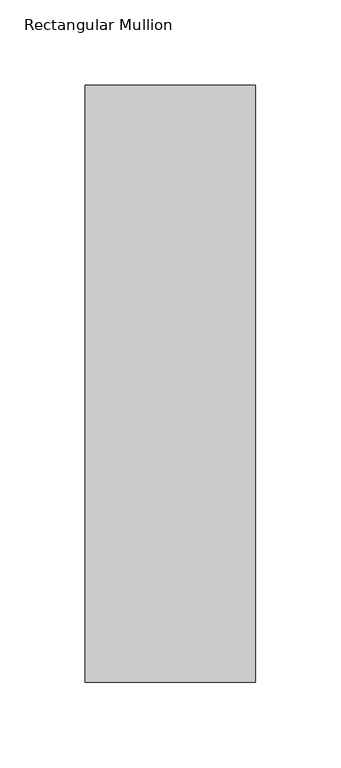
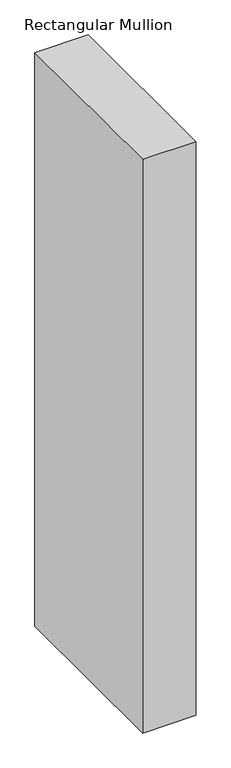
"""IFC4 building model written with IfcOpenShell, lengths in millimetres: member geometry, Rectangular Mullion : WWm-100x350-100mmOffset."""

import ifcopenshell
import ifcopenshell.guid

model = None  # the IFC model being written
_history = None  # IfcOwnerHistory: only IFC2X3 demands one
_inside = {}  # id of a spatial element -> (the spatial element, [elements in it])
_under = {}  # id of a project, library or spatial element -> (it, [spatial elements below it])
_declared = {}  # id of a project -> (the project, [libraries it declares])
_typed = {}  # id of a type object -> (the type object, [elements of that type])
_made_of = {}  # id of a material, layer set ... -> (it, [elements and type objects made of it])


def new_model(schema):
    """Start an empty IFC model of exactly this schema.

    Asked for "IFC4X3", IfcOpenShell would pick the latest addendum, in which some entities
    have other attributes; the version numbers below select the first issue.
    IFC2X3 requires an IfcOwnerHistory on every rooted entity: one is made here for all.
    """
    global model, _history
    if schema == "IFC4X3":
        model = ifcopenshell.file(schema_version=(4, 3, 0, 0))
    else:
        model = ifcopenshell.file(schema=schema)
    _inside.clear()
    _under.clear()
    _declared.clear()
    _typed.clear()
    _made_of.clear()
    _history = None
    if model.schema == "IFC2X3":
        org = make("IfcOrganization", Name="unknown")
        user = make(
            "IfcPersonAndOrganization",
            ThePerson=make("IfcPerson", FamilyName="unknown"),
            TheOrganization=org,
        )
        app = make(
            "IfcApplication",
            ApplicationDeveloper=org,
            Version="unknown",
            ApplicationFullName="unknown",
            ApplicationIdentifier="unknown",
        )
        _history = make(
            "IfcOwnerHistory",
            OwningUser=user,
            OwningApplication=app,
            ChangeAction="ADDED",
            CreationDate=0,
        )
    return model


def make(cls, **values):
    """One entity of the class cls with the attributes given. An attribute that is None is left unset."""
    return model.create_entity(
        cls, **{name: value for name, value in values.items() if value is not None}
    )


def rooted(cls, **values):
    """An entity with a GlobalId (a new one), such as an element, a storey or a relation."""
    return make(cls, GlobalId=ifcopenshell.guid.new(), OwnerHistory=_history, **values)


def si_unit(unit_type, name, prefix=None):
    """IfcSIUnit, for example si_unit("LENGTHUNIT", "METRE", prefix="MILLI")."""
    return make("IfcSIUnit", UnitType=unit_type, Prefix=prefix, Name=name)


def assignment(units):
    """IfcUnitAssignment: the units of a project."""
    return None if units is None else make("IfcUnitAssignment", Units=units)


def point(xyz):
    """IfcCartesianPoint."""
    return None if xyz is None else make("IfcCartesianPoint", Coordinates=xyz)


def direction(xyz):
    """IfcDirection."""
    return None if xyz is None else make("IfcDirection", DirectionRatios=xyz)


def frame(location, z_axis=None, x_axis=None):
    """IfcAxis2Placement3D, a coordinate frame: its origin and axes. An axis left out is left unset."""
    return make(
        "IfcAxis2Placement3D",
        Location=point(location),
        Axis=direction(z_axis),
        RefDirection=direction(x_axis),
    )


def origin():
    """The frame at (0, 0, 0) with its axes left unset."""
    return frame((0.0, 0.0, 0.0))


def place(relative_to, where):
    """IfcLocalPlacement: puts the frame where relative to a parent placement (None: the world)."""
    return make(
        "IfcLocalPlacement", PlacementRelTo=relative_to, RelativePlacement=where
    )


def context(
    kind, dimensions, precision=None, world=None, true_north=None, identifier=None
):
    """IfcGeometricRepresentationContext, for example the 3D "Model" context."""
    return make(
        "IfcGeometricRepresentationContext",
        ContextIdentifier=identifier,
        ContextType=kind,
        CoordinateSpaceDimension=dimensions,
        Precision=precision,
        WorldCoordinateSystem=world,
        TrueNorth=true_north,
    )


def project(units=None, contexts=None):
    """IfcProject with its units and contexts."""
    return rooted(
        "IfcProject",
        Name="project",
        RepresentationContexts=contexts,
        UnitsInContext=assignment(units),
    )


def spatial(cls, under=None, at=None, **own):
    """A site, building, storey or space (cls), placed at a placement, below another one or the project."""
    s = rooted(cls, ObjectPlacement=at, **own)
    if under is not None:
        _under.setdefault(under.id(), (under, []))[1].append(s)
    return s


def polyline(points):
    """IfcPolyline through the points."""
    return make("IfcPolyline", Points=[point(p) for p in points])


def outline(outer, holes=None, kind="AREA"):
    """IfcArbitraryClosedProfileDef: a profile drawn as a closed curve; with holes, ...WithVoids."""
    if holes is None:
        return make("IfcArbitraryClosedProfileDef", ProfileType=kind, OuterCurve=outer)
    return make(
        "IfcArbitraryProfileDefWithVoids",
        ProfileType=kind,
        OuterCurve=outer,
        InnerCurves=holes,
    )


def extrude(swept, where, along, depth):
    """IfcExtrudedAreaSolid: the profile swept, set in the frame where, extruded along a direction by depth."""
    return make(
        "IfcExtrudedAreaSolid",
        SweptArea=swept,
        Position=where,
        ExtrudedDirection=direction(along),
        Depth=depth,
    )


def shape(context_of_items, identifier, shape_type, items):
    """IfcShapeRepresentation: the items that make up one representation, for example the "Body"."""
    return make(
        "IfcShapeRepresentation",
        ContextOfItems=context_of_items,
        RepresentationIdentifier=identifier,
        RepresentationType=shape_type,
        Items=items,
    )


def source(mapping_origin, context_of_items, identifier, shape_type, items):
    """IfcRepresentationMap: a shape defined once, which mapped items show again and again."""
    return make(
        "IfcRepresentationMap",
        MappingOrigin=mapping_origin,
        MappedRepresentation=shape(context_of_items, identifier, shape_type, items),
    )


def transform(
    local_origin,
    x_axis=None,
    y_axis=None,
    z_axis=None,
    scale=None,
    scale2=None,
    scale3=None,
    uniform=True,
):
    """IfcCartesianTransformationOperator3D, or its non-uniform kind. x_axis, y_axis, z_axis: its Axis1, 2, 3."""
    if uniform:
        return make(
            "IfcCartesianTransformationOperator3D",
            Axis1=direction(x_axis),
            Axis2=direction(y_axis),
            LocalOrigin=point(local_origin),
            Scale=scale,
            Axis3=direction(z_axis),
        )
    return make(
        "IfcCartesianTransformationOperator3DnonUniform",
        Axis1=direction(x_axis),
        Axis2=direction(y_axis),
        LocalOrigin=point(local_origin),
        Scale=scale,
        Axis3=direction(z_axis),
        Scale2=scale2,
        Scale3=scale3,
    )


def mapped(mapping_source, mapping_target):
    """IfcMappedItem: shows the shape of a source again, moved by a transform."""
    return make(
        "IfcMappedItem", MappingSource=mapping_source, MappingTarget=mapping_target
    )


def made_of(thing, what):
    """Note that an element or type object is made of a material, layer set ...; save() writes the relation."""
    if what is not None:
        _made_of.setdefault(what.id(), (what, []))[1].append(thing)
    return thing


def element(
    cls,
    number,
    at=None,
    inside=None,
    cuts=None,
    type_object=None,
    material=None,
    context=None,
    identifier="Body",
    shape_type=None,
    held_by="IfcProductDefinitionShape",
    body=None,
    shapes=None,
    **own,
):
    """One element of the class cls, such as IfcWall. Its Tag is "e" and its number.

    at: its placement. inside: the storey or other place that contains it. cuts: it is an
    opening in that element (IfcRelVoidsElement). A single representation is given by context,
    identifier, shape_type and body (its items); several are given by shapes. held_by: the class
    of the entity that holds the representations. save() writes the other relations.
    """
    e = rooted(cls, Tag="e%d" % number, ObjectPlacement=at, **own)
    if body is not None:
        shapes = [shape(context, identifier, shape_type, body)]
    if shapes is not None:
        e.Representation = make(held_by, Representations=shapes)
    if inside is not None:
        _inside.setdefault(inside.id(), (inside, []))[1].append(e)
    if cuts is not None:
        rooted(
            "IfcRelVoidsElement", RelatingBuildingElement=cuts, RelatedOpeningElement=e
        )
    if type_object is not None:
        _typed.setdefault(type_object.id(), (type_object, []))[1].append(e)
    return made_of(e, material)


def aggregate(whole, parts):
    """IfcRelAggregates: a whole, such as a stair, and the parts it consists of."""
    return rooted("IfcRelAggregates", RelatingObject=whole, RelatedObjects=parts)


def save(model, path):
    """Write the relations noted so far, then the file.

    IfcRelAggregates (storeys below a building ...), IfcRelContainedInSpatialStructure (elements
    in a storey), IfcRelDefinesByType, IfcRelAssociatesMaterial and IfcRelDeclares: one each for
    every whole, place, type object, material and project.
    """
    for whole, parts in _under.values():
        aggregate(whole, parts)
    for where, things in _inside.values():
        rooted(
            "IfcRelContainedInSpatialStructure",
            RelatedElements=things,
            RelatingStructure=where,
        )
    for kind, things in _typed.values():
        rooted("IfcRelDefinesByType", RelatedObjects=things, RelatingType=kind)
    for what, things in _made_of.values():
        rooted("IfcRelAssociatesMaterial", RelatedObjects=things, RelatingMaterial=what)
    for by, libraries in _declared.values():
        rooted("IfcRelDeclares", RelatingContext=by, RelatedDefinitions=libraries)
    model.write(path)


def rectangular_mullion_18d69dd7(model_context):
    return source(origin(), model_context, "Body", "SweptSolid", [
        extrude(outline(polyline([(0.0, 175.0), (0.0, -175.0), (-100.0, -175.0), (-100.0, 175.0), (0.0, 175.0)])), frame((0.0, 0.0, -1138.7692613), z_axis=(0.0, 0.0, 1.0), x_axis=(1.0, 0.0, 0.0)), (0.0, 0.0, 1.0), 1138.7692613),
    ])


if __name__ == "__main__":
    model = new_model("IFC4")
    model_context = context("Model", 3, world=origin())
    ifc_project = project(units=[si_unit("LENGTHUNIT", "METRE", prefix="MILLI")], contexts=[model_context])
    site = spatial("IfcSite", under=ifc_project)
    building = spatial("IfcBuilding", under=site)
    placement = place(None, origin())
    rectangular_mullion_shape = rectangular_mullion_18d69dd7(model_context)
    element("IfcMember", 1, ObjectType="Rectangular Mullion : WWm-100x350-100mmOffset", at=placement, inside=building, context=model_context, shape_type="MappedRepresentation", body=[
        mapped(rectangular_mullion_shape, transform((0.0, 0.0, 0.0), x_axis=(1.0, 0.0, 0.0), y_axis=(0.0, 1.0, 0.0), z_axis=(0.0, 0.0, 1.0))),
    ])
    save(model, "model.ifc")

# Revit data of these elements
# Type "Rectangular Mullion : WWm-100x350-100mmOffset"
#   built-in parameter 1007304 = 1.14829 (stored number, unit not read)
#   built-in parameter 1007301 = 0.164042 (stored number, unit not read)
#   built-in parameter 1007300 = 0.164042 (stored number, unit not read)
# Element 1 (IfcMember, "Rectangular Mullion : WWm-100x350-100mmOffset")
#   Materials on its faces: "WW-EC-RGB-Mullion"
# Materials
#   "WW-EC-RGB-Mullion": class "Generic", colour RGB 255 255 255, transparency 0, Comments = "If region requests black mullions, switch asset color to RGB 25-25-25", Description = "Generic Color", Cost = 0
